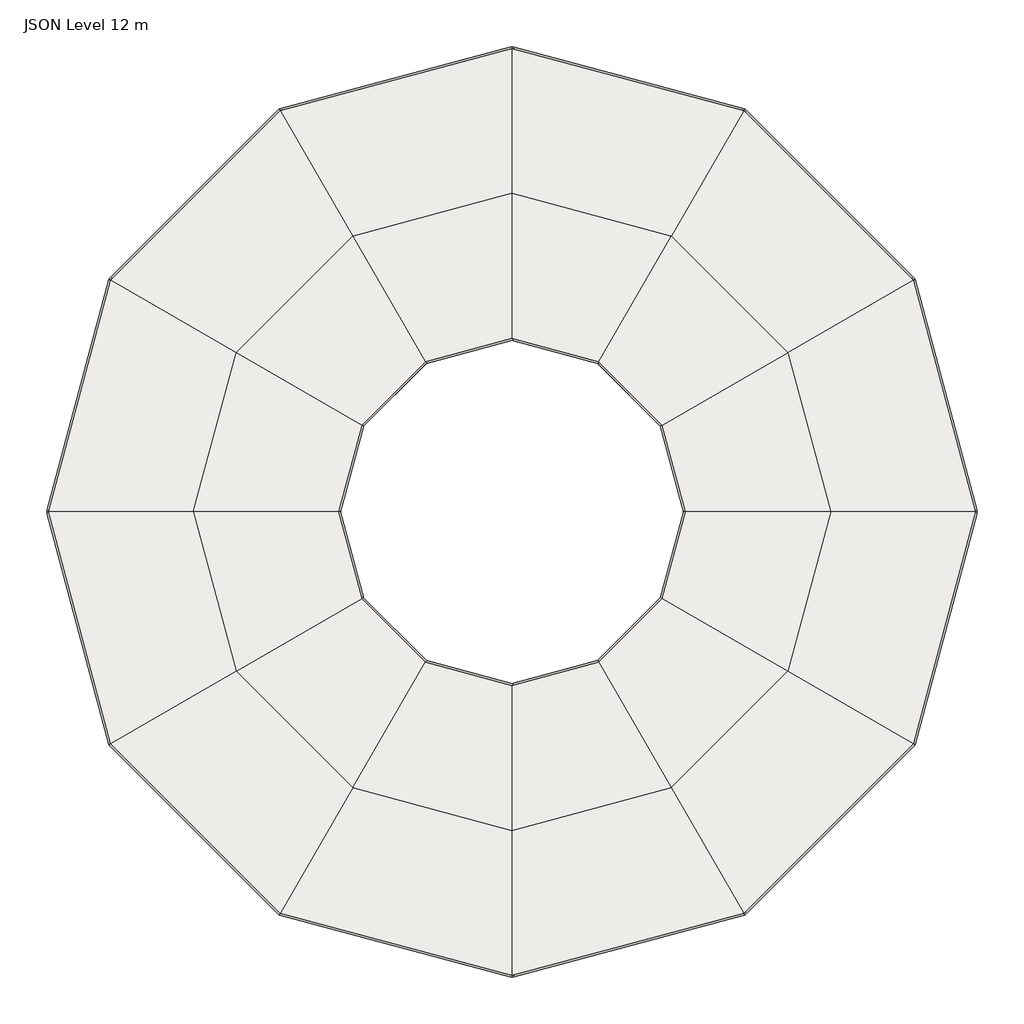
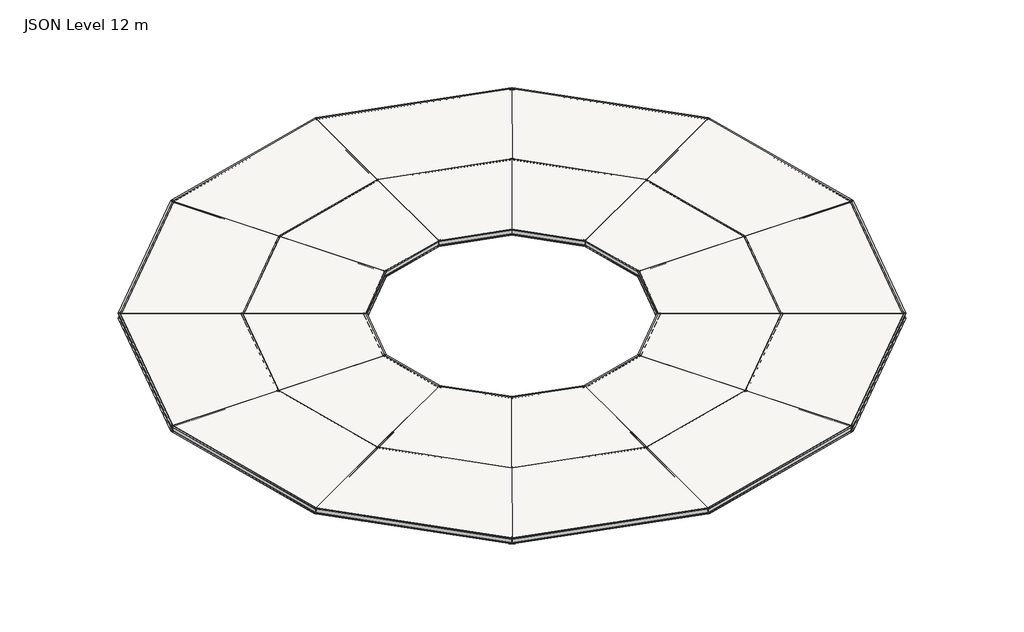
# One storey: 60 beams, 24 slabs.
"""IFC4 building model written with IfcOpenShell, lengths in millimetres."""

import ifcopenshell
import ifcopenshell.guid

model = None  # the IFC model being written
_history = None  # IfcOwnerHistory: only IFC2X3 demands one
_inside = {}  # id of a spatial element -> (the spatial element, [elements in it])
_under = {}  # id of a project, library or spatial element -> (it, [spatial elements below it])
_declared = {}  # id of a project -> (the project, [libraries it declares])
_typed = {}  # id of a type object -> (the type object, [elements of that type])
_made_of = {}  # id of a material, layer set ... -> (it, [elements and type objects made of it])


def new_model(schema):
    """Start an empty IFC model of exactly this schema.

    Asked for "IFC4X3", IfcOpenShell would pick the latest addendum, in which some entities
    have other attributes; the version numbers below select the first issue.
    IFC2X3 requires an IfcOwnerHistory on every rooted entity: one is made here for all.
    """
    global model, _history
    if schema == "IFC4X3":
        model = ifcopenshell.file(schema_version=(4, 3, 0, 0))
    else:
        model = ifcopenshell.file(schema=schema)
    _inside.clear()
    _under.clear()
    _declared.clear()
    _typed.clear()
    _made_of.clear()
    _history = None
    if model.schema == "IFC2X3":
        org = make("IfcOrganization", Name="unknown")
        user = make(
            "IfcPersonAndOrganization",
            ThePerson=make("IfcPerson", FamilyName="unknown"),
            TheOrganization=org,
        )
        app = make(
            "IfcApplication",
            ApplicationDeveloper=org,
            Version="unknown",
            ApplicationFullName="unknown",
            ApplicationIdentifier="unknown",
        )
        _history = make(
            "IfcOwnerHistory",
            OwningUser=user,
            OwningApplication=app,
            ChangeAction="ADDED",
            CreationDate=0,
        )
    return model


def make(cls, **values):
    """One entity of the class cls with the attributes given. An attribute that is None is left unset."""
    return model.create_entity(
        cls, **{name: value for name, value in values.items() if value is not None}
    )


def rooted(cls, **values):
    """An entity with a GlobalId (a new one), such as an element, a storey or a relation."""
    return make(cls, GlobalId=ifcopenshell.guid.new(), OwnerHistory=_history, **values)


def si_unit(unit_type, name, prefix=None):
    """IfcSIUnit, for example si_unit("LENGTHUNIT", "METRE", prefix="MILLI")."""
    return make("IfcSIUnit", UnitType=unit_type, Prefix=prefix, Name=name)


def assignment(units):
    """IfcUnitAssignment: the units of a project."""
    return None if units is None else make("IfcUnitAssignment", Units=units)


def point(xyz):
    """IfcCartesianPoint."""
    return None if xyz is None else make("IfcCartesianPoint", Coordinates=xyz)


def direction(xyz):
    """IfcDirection."""
    return None if xyz is None else make("IfcDirection", DirectionRatios=xyz)


def frame(location, z_axis=None, x_axis=None):
    """IfcAxis2Placement3D, a coordinate frame: its origin and axes. An axis left out is left unset."""
    return make(
        "IfcAxis2Placement3D",
        Location=point(location),
        Axis=direction(z_axis),
        RefDirection=direction(x_axis),
    )


def frame_2d(location, x_axis=None):
    """IfcAxis2Placement2D, a coordinate frame in the plane: its origin and x axis."""
    return make(
        "IfcAxis2Placement2D", Location=point(location), RefDirection=direction(x_axis)
    )


def origin():
    """The frame at (0, 0, 0) with its axes left unset."""
    return frame((0.0, 0.0, 0.0))


def place(relative_to, where):
    """IfcLocalPlacement: puts the frame where relative to a parent placement (None: the world)."""
    return make(
        "IfcLocalPlacement", PlacementRelTo=relative_to, RelativePlacement=where
    )


def context(
    kind, dimensions, precision=None, world=None, true_north=None, identifier=None
):
    """IfcGeometricRepresentationContext, for example the 3D "Model" context."""
    return make(
        "IfcGeometricRepresentationContext",
        ContextIdentifier=identifier,
        ContextType=kind,
        CoordinateSpaceDimension=dimensions,
        Precision=precision,
        WorldCoordinateSystem=world,
        TrueNorth=true_north,
    )


def project(units=None, contexts=None):
    """IfcProject with its units and contexts."""
    return rooted(
        "IfcProject",
        Name="project",
        RepresentationContexts=contexts,
        UnitsInContext=assignment(units),
    )


def spatial(cls, under=None, at=None, **own):
    """A site, building, storey or space (cls), placed at a placement, below another one or the project."""
    s = rooted(cls, ObjectPlacement=at, **own)
    if under is not None:
        _under.setdefault(under.id(), (under, []))[1].append(s)
    return s


def polyline(points):
    """IfcPolyline through the points."""
    return make("IfcPolyline", Points=[point(p) for p in points])


def circle_curve(where, radius):
    """IfcCircle in the frame where."""
    return make("IfcCircle", Position=where, Radius=radius)


def trimmed(basis, trim1, trim2, sense, master):
    """IfcTrimmedCurve: the piece of a basis curve between two trims."""
    return make(
        "IfcTrimmedCurve",
        BasisCurve=basis,
        Trim1=trim1,
        Trim2=trim2,
        SenseAgreement=sense,
        MasterRepresentation=master,
    )


def segment(curve, same_sense, transition):
    """IfcCompositeCurveSegment."""
    return make(
        "IfcCompositeCurveSegment",
        Transition=transition,
        SameSense=same_sense,
        ParentCurve=curve,
    )


def composite_curve(segments, self_intersect=None):
    """IfcCompositeCurve: segments joined end to end."""
    return make("IfcCompositeCurve", Segments=segments, SelfIntersect=self_intersect)


def outline(outer, holes=None, kind="AREA"):
    """IfcArbitraryClosedProfileDef: a profile drawn as a closed curve; with holes, ...WithVoids."""
    if holes is None:
        return make("IfcArbitraryClosedProfileDef", ProfileType=kind, OuterCurve=outer)
    return make(
        "IfcArbitraryProfileDefWithVoids",
        ProfileType=kind,
        OuterCurve=outer,
        InnerCurves=holes,
    )


def extrude(swept, where, along, depth):
    """IfcExtrudedAreaSolid: the profile swept, set in the frame where, extruded along a direction by depth."""
    return make(
        "IfcExtrudedAreaSolid",
        SweptArea=swept,
        Position=where,
        ExtrudedDirection=direction(along),
        Depth=depth,
    )


def shape(context_of_items, identifier, shape_type, items):
    """IfcShapeRepresentation: the items that make up one representation, for example the "Body"."""
    return make(
        "IfcShapeRepresentation",
        ContextOfItems=context_of_items,
        RepresentationIdentifier=identifier,
        RepresentationType=shape_type,
        Items=items,
    )


def source(mapping_origin, context_of_items, identifier, shape_type, items):
    """IfcRepresentationMap: a shape defined once, which mapped items show again and again."""
    return make(
        "IfcRepresentationMap",
        MappingOrigin=mapping_origin,
        MappedRepresentation=shape(context_of_items, identifier, shape_type, items),
    )


def transform(
    local_origin,
    x_axis=None,
    y_axis=None,
    z_axis=None,
    scale=None,
    scale2=None,
    scale3=None,
    uniform=True,
):
    """IfcCartesianTransformationOperator3D, or its non-uniform kind. x_axis, y_axis, z_axis: its Axis1, 2, 3."""
    if uniform:
        return make(
            "IfcCartesianTransformationOperator3D",
            Axis1=direction(x_axis),
            Axis2=direction(y_axis),
            LocalOrigin=point(local_origin),
            Scale=scale,
            Axis3=direction(z_axis),
        )
    return make(
        "IfcCartesianTransformationOperator3DnonUniform",
        Axis1=direction(x_axis),
        Axis2=direction(y_axis),
        LocalOrigin=point(local_origin),
        Scale=scale,
        Axis3=direction(z_axis),
        Scale2=scale2,
        Scale3=scale3,
    )


def mapped(mapping_source, mapping_target):
    """IfcMappedItem: shows the shape of a source again, moved by a transform."""
    return make(
        "IfcMappedItem", MappingSource=mapping_source, MappingTarget=mapping_target
    )


def made_of(thing, what):
    """Note that an element or type object is made of a material, layer set ...; save() writes the relation."""
    if what is not None:
        _made_of.setdefault(what.id(), (what, []))[1].append(thing)
    return thing


def element(
    cls,
    number,
    at=None,
    inside=None,
    cuts=None,
    type_object=None,
    material=None,
    context=None,
    identifier="Body",
    shape_type=None,
    held_by="IfcProductDefinitionShape",
    body=None,
    shapes=None,
    **own,
):
    """One element of the class cls, such as IfcWall. Its Tag is "e" and its number.

    at: its placement. inside: the storey or other place that contains it. cuts: it is an
    opening in that element (IfcRelVoidsElement). A single representation is given by context,
    identifier, shape_type and body (its items); several are given by shapes. held_by: the class
    of the entity that holds the representations. save() writes the other relations.
    """
    e = rooted(cls, Tag="e%d" % number, ObjectPlacement=at, **own)
    if body is not None:
        shapes = [shape(context, identifier, shape_type, body)]
    if shapes is not None:
        e.Representation = make(held_by, Representations=shapes)
    if inside is not None:
        _inside.setdefault(inside.id(), (inside, []))[1].append(e)
    if cuts is not None:
        rooted(
            "IfcRelVoidsElement", RelatingBuildingElement=cuts, RelatedOpeningElement=e
        )
    if type_object is not None:
        _typed.setdefault(type_object.id(), (type_object, []))[1].append(e)
    return made_of(e, material)


def aggregate(whole, parts):
    """IfcRelAggregates: a whole, such as a stair, and the parts it consists of."""
    return rooted("IfcRelAggregates", RelatingObject=whole, RelatedObjects=parts)


def save(model, path):
    """Write the relations noted so far, then the file.

    IfcRelAggregates (storeys below a building ...), IfcRelContainedInSpatialStructure (elements
    in a storey), IfcRelDefinesByType, IfcRelAssociatesMaterial and IfcRelDeclares: one each for
    every whole, place, type object, material and project.
    """
    for whole, parts in _under.values():
        aggregate(whole, parts)
    for where, things in _inside.values():
        rooted(
            "IfcRelContainedInSpatialStructure",
            RelatedElements=things,
            RelatingStructure=where,
        )
    for kind, things in _typed.values():
        rooted("IfcRelDefinesByType", RelatedObjects=things, RelatingType=kind)
    for what, things in _made_of.values():
        rooted("IfcRelAssociatesMaterial", RelatedObjects=things, RelatingMaterial=what)
    for by, libraries in _declared.values():
        rooted("IfcRelDeclares", RelatingContext=by, RelatedDefinitions=libraries)
    model.write(path)


def ub_universal_beams_ub254x146x31_beafa172(model_context):
    return source(origin(), model_context, "Body", "SweptSolid", [
        extrude(outline(composite_curve([segment(polyline([(73.05, -117.1), (73.05, -125.7), (-73.05, -125.7), (-73.05, -117.1), (-10.6, -117.1)]), True, "CONTINUOUS"), segment(trimmed(circle_curve(frame_2d((-10.6, -109.5)), 7.6), [point((-10.6, -117.1))], [point((-3.0, -109.5))], True, "CARTESIAN"), True, "CONTINUOUS"), segment(polyline([(-3.0, -109.5), (-3.0, 109.5)]), True, "CONTINUOUS"), segment(trimmed(circle_curve(frame_2d((-10.6, 109.5)), 7.6), [point((-3.0, 109.5))], [point((-10.6, 117.1))], True, "CARTESIAN"), True, "CONTINUOUS"), segment(polyline([(-10.6, 117.1), (-73.05, 117.1), (-73.05, 125.7), (73.05, 125.7), (73.05, 117.1), (10.6, 117.1)]), True, "CONTINUOUS"), segment(trimmed(circle_curve(frame_2d((10.6, 109.5)), 7.6), [point((10.6, 117.1))], [point((3.0, 109.5))], True, "CARTESIAN"), True, "CONTINUOUS"), segment(polyline([(3.0, 109.5), (3.0, -109.5)]), True, "CONTINUOUS"), segment(trimmed(circle_curve(frame_2d((10.6, -109.5)), 7.6), [point((3.0, -109.5))], [point((10.6, -117.1))], True, "CARTESIAN"), True, "CONTINUOUS"), segment(polyline([(10.6, -117.1), (73.05, -117.1)]), True, "CONTINUOUS")], self_intersect=False)), frame((-1552.9, 0.0, 0.0), z_axis=(1.0, 0.0, 0.0), x_axis=(0.0, 1.0, 0.0)), (0.0, 0.0, 1.0), 3105.8),
    ])


def ub_universal_beams_ub254x146x31_048477c2(model_context):
    return source(origin(), model_context, "Body", "SweptSolid", [
        extrude(outline(composite_curve([segment(polyline([(73.05, -117.1), (73.05, -125.7), (-73.05, -125.7), (-73.05, -117.1), (-10.6, -117.1)]), True, "CONTINUOUS"), segment(trimmed(circle_curve(frame_2d((-10.6, -109.5)), 7.6), [point((-10.6, -117.1))], [point((-3.0, -109.5))], True, "CARTESIAN"), True, "CONTINUOUS"), segment(polyline([(-3.0, -109.5), (-3.0, 109.5)]), True, "CONTINUOUS"), segment(trimmed(circle_curve(frame_2d((-10.6, 109.5)), 7.6), [point((-3.0, 109.5))], [point((-10.6, 117.1))], True, "CARTESIAN"), True, "CONTINUOUS"), segment(polyline([(-10.6, 117.1), (-73.05, 117.1), (-73.05, 125.7), (73.05, 125.7), (73.05, 117.1), (10.6, 117.1)]), True, "CONTINUOUS"), segment(trimmed(circle_curve(frame_2d((10.6, 109.5)), 7.6), [point((10.6, 117.1))], [point((3.0, 109.5))], True, "CARTESIAN"), True, "CONTINUOUS"), segment(polyline([(3.0, 109.5), (3.0, -109.5)]), True, "CONTINUOUS"), segment(trimmed(circle_curve(frame_2d((10.6, -109.5)), 7.6), [point((3.0, -109.5))], [point((10.6, -117.1))], True, "CARTESIAN"), True, "CONTINUOUS"), segment(polyline([(10.6, -117.1), (73.05, -117.1)]), True, "CONTINUOUS")], self_intersect=False)), frame((-2847.0, 0.0, 0.0), z_axis=(1.0, 0.0, 0.0), x_axis=(0.0, 1.0, 0.0)), (0.0, 0.0, 1.0), 5694.0),
    ])


def ub_universal_beams_ub254x146x31_9e4386c4(model_context):
    return source(origin(), model_context, "Body", "SweptSolid", [
        extrude(outline(composite_curve([segment(polyline([(73.05, -117.1), (73.05, -125.7), (-73.05, -125.7), (-73.05, -117.1), (-10.6, -117.1)]), True, "CONTINUOUS"), segment(trimmed(circle_curve(frame_2d((-10.6, -109.5)), 7.6), [point((-10.6, -117.1))], [point((-3.0, -109.5))], True, "CARTESIAN"), True, "CONTINUOUS"), segment(polyline([(-3.0, -109.5), (-3.0, 109.5)]), True, "CONTINUOUS"), segment(trimmed(circle_curve(frame_2d((-10.6, 109.5)), 7.6), [point((-3.0, 109.5))], [point((-10.6, 117.1))], True, "CARTESIAN"), True, "CONTINUOUS"), segment(polyline([(-10.6, 117.1), (-73.05, 117.1), (-73.05, 125.7), (73.05, 125.7), (73.05, 117.1), (10.6, 117.1)]), True, "CONTINUOUS"), segment(trimmed(circle_curve(frame_2d((10.6, 109.5)), 7.6), [point((10.6, 117.1))], [point((3.0, 109.5))], True, "CARTESIAN"), True, "CONTINUOUS"), segment(polyline([(3.0, 109.5), (3.0, -109.5)]), True, "CONTINUOUS"), segment(trimmed(circle_curve(frame_2d((10.6, -109.5)), 7.6), [point((3.0, -109.5))], [point((10.6, -117.1))], True, "CARTESIAN"), True, "CONTINUOUS"), segment(polyline([(10.6, -117.1), (73.05, -117.1)]), True, "CONTINUOUS")], self_intersect=False)), frame((-4141.1, 0.0, 0.0), z_axis=(1.0, 0.0, 0.0), x_axis=(0.0, 1.0, 0.0)), (0.0, 0.0, 1.0), 8282.2),
    ])


def ub_universal_beams_ub254x146x31_ce116be2(model_context):
    return source(origin(), model_context, "Body", "SweptSolid", [
        extrude(outline(composite_curve([segment(polyline([(73.05, -117.1), (73.05, -125.7), (-73.05, -125.7), (-73.05, -117.1), (-10.6, -117.1)]), True, "CONTINUOUS"), segment(trimmed(circle_curve(frame_2d((-10.6, -109.5)), 7.6), [point((-10.6, -117.1))], [point((-3.0, -109.5))], True, "CARTESIAN"), True, "CONTINUOUS"), segment(polyline([(-3.0, -109.5), (-3.0, 109.5)]), True, "CONTINUOUS"), segment(trimmed(circle_curve(frame_2d((-10.6, 109.5)), 7.6), [point((-3.0, 109.5))], [point((-10.6, 117.1))], True, "CARTESIAN"), True, "CONTINUOUS"), segment(polyline([(-10.6, 117.1), (-73.05, 117.1), (-73.05, 125.7), (73.05, 125.7), (73.05, 117.1), (10.6, 117.1)]), True, "CONTINUOUS"), segment(trimmed(circle_curve(frame_2d((10.6, 109.5)), 7.6), [point((10.6, 117.1))], [point((3.0, 109.5))], True, "CARTESIAN"), True, "CONTINUOUS"), segment(polyline([(3.0, 109.5), (3.0, -109.5)]), True, "CONTINUOUS"), segment(trimmed(circle_curve(frame_2d((10.6, -109.5)), 7.6), [point((3.0, -109.5))], [point((10.6, -117.1))], True, "CARTESIAN"), True, "CONTINUOUS"), segment(polyline([(10.6, -117.1), (73.05, -117.1)]), True, "CONTINUOUS")], self_intersect=False)), frame((-2500.0, 0.0, 0.0), z_axis=(1.0, 0.0, 0.0), x_axis=(0.0, 1.0, 0.0)), (0.0, 0.0, 1.0), 5000.0),
    ])


model = new_model("IFC4")

# Units and contexts
model_context = context("Model", 3, world=origin())
ifc_project = project(units=[si_unit("LENGTHUNIT", "METRE", prefix="MILLI")], contexts=[model_context])

# Site, building, storey
site = spatial("IfcSite", under=ifc_project)
building = spatial("IfcBuilding", under=site)
storey = spatial("IfcBuildingStorey", under=building, Name="JSON Level 12 m", Elevation=12000.0)

# Beams
placement = place(None, origin())
ub_universal_beams_ub254x146x31_shape = ub_universal_beams_ub254x146x31_beafa172(model_context)
element("IfcBeam", 1, ObjectType="UB-Universal Beams : UB254x146x31", at=placement, inside=storey, context=model_context, shape_type="MappedRepresentation", body=[
    mapped(ub_universal_beams_ub254x146x31_shape, transform((5598.0762114, 1500.0, 11874.3), x_axis=(-0.2588190451025206, 0.9659258262890683, 0.0), y_axis=(-0.9659258262890683, -0.2588190451025206, 0.0), z_axis=(0.0, 0.0, 1.0))),
])
element("IfcBeam", 2, ObjectType="UB-Universal Beams : UB254x146x31", at=placement, inside=storey, context=model_context, shape_type="MappedRepresentation", body=[
    mapped(ub_universal_beams_ub254x146x31_shape, transform((4098.0762114, 4098.0762114, 11874.3), x_axis=(-0.7071067811865472, 0.7071067811865477, 0.0), y_axis=(-0.7071067811865477, -0.7071067811865472, 0.0), z_axis=(0.0, 0.0, 1.0))),
])
element("IfcBeam", 3, ObjectType="UB-Universal Beams : UB254x146x31", at=placement, inside=storey, context=model_context, shape_type="MappedRepresentation", body=[
    mapped(ub_universal_beams_ub254x146x31_shape, transform((1500.0, 5598.0762114, 11874.3), x_axis=(-0.9659258262890683, 0.2588190451025205, 0.0), y_axis=(-0.2588190451025205, -0.9659258262890683, 0.0), z_axis=(0.0, 0.0, 1.0))),
])
element("IfcBeam", 4, ObjectType="UB-Universal Beams : UB254x146x31", at=placement, inside=storey, context=model_context, shape_type="MappedRepresentation", body=[
    mapped(ub_universal_beams_ub254x146x31_shape, transform((-1500.0, 5598.0762114, 11874.3), x_axis=(-0.9659258262890683, -0.2588190451025206, 0.0), y_axis=(0.2588190451025206, -0.9659258262890683, 0.0), z_axis=(0.0, 0.0, 1.0))),
])
element("IfcBeam", 5, ObjectType="UB-Universal Beams : UB254x146x31", at=placement, inside=storey, context=model_context, shape_type="MappedRepresentation", body=[
    mapped(ub_universal_beams_ub254x146x31_shape, transform((-4098.0762114, 4098.0762114, 11874.3), x_axis=(-0.7071067811865477, -0.7071067811865475, 0.0), y_axis=(0.7071067811865475, -0.7071067811865477, 0.0), z_axis=(0.0, 0.0, 1.0))),
])
element("IfcBeam", 6, ObjectType="UB-Universal Beams : UB254x146x31", at=placement, inside=storey, context=model_context, shape_type="MappedRepresentation", body=[
    mapped(ub_universal_beams_ub254x146x31_shape, transform((-5598.0762114, 1500.0, 11874.3), x_axis=(-0.25881904510252063, -0.9659258262890683, 0.0), y_axis=(0.9659258262890683, -0.25881904510252063, 0.0), z_axis=(0.0, 0.0, 1.0))),
])
element("IfcBeam", 7, ObjectType="UB-Universal Beams : UB254x146x31", at=placement, inside=storey, context=model_context, shape_type="MappedRepresentation", body=[
    mapped(ub_universal_beams_ub254x146x31_shape, transform((-5598.0762114, -1500.0, 11874.3), x_axis=(0.25881904510252035, -0.9659258262890685, 0.0), y_axis=(0.9659258262890685, 0.25881904510252035, 0.0), z_axis=(0.0, 0.0, 1.0))),
])
element("IfcBeam", 8, ObjectType="UB-Universal Beams : UB254x146x31", at=placement, inside=storey, context=model_context, shape_type="MappedRepresentation", body=[
    mapped(ub_universal_beams_ub254x146x31_shape, transform((-4098.0762114, -4098.0762114, 11874.3), x_axis=(0.7071067811865471, -0.7071067811865478, 0.0), y_axis=(0.7071067811865478, 0.7071067811865471, 0.0), z_axis=(0.0, 0.0, 1.0))),
])
element("IfcBeam", 9, ObjectType="UB-Universal Beams : UB254x146x31", at=placement, inside=storey, context=model_context, shape_type="MappedRepresentation", body=[
    mapped(ub_universal_beams_ub254x146x31_shape, transform((-1500.0, -5598.0762114, 11874.3), x_axis=(0.9659258262890682, -0.25881904510252074, 0.0), y_axis=(0.25881904510252074, 0.9659258262890682, 0.0), z_axis=(0.0, 0.0, 1.0))),
])
element("IfcBeam", 10, ObjectType="UB-Universal Beams : UB254x146x31", at=placement, inside=storey, context=model_context, shape_type="MappedRepresentation", body=[
    mapped(ub_universal_beams_ub254x146x31_shape, transform((1500.0, -5598.0762114, 11874.3), x_axis=(0.9659258262890684, 0.25881904510252035, 0.0), y_axis=(-0.25881904510252035, 0.9659258262890684, 0.0), z_axis=(0.0, 0.0, 1.0))),
])
element("IfcBeam", 11, ObjectType="UB-Universal Beams : UB254x146x31", at=placement, inside=storey, context=model_context, shape_type="MappedRepresentation", body=[
    mapped(ub_universal_beams_ub254x146x31_shape, transform((4098.0762114, -4098.0762114, 11874.3), x_axis=(0.7071067811865474, 0.7071067811865476, 0.0), y_axis=(-0.7071067811865476, 0.7071067811865474, 0.0), z_axis=(0.0, 0.0, 1.0))),
])
element("IfcBeam", 12, ObjectType="UB-Universal Beams : UB254x146x31", at=placement, inside=storey, context=model_context, shape_type="MappedRepresentation", body=[
    mapped(ub_universal_beams_ub254x146x31_shape, transform((5598.0762114, -1500.0, 11874.3), x_axis=(0.25881904510252096, 0.9659258262890682, 0.0), y_axis=(-0.9659258262890682, 0.25881904510252096, 0.0), z_axis=(0.0, 0.0, 1.0))),
])
ub_universal_beams_ub254x146x31_2_shape = ub_universal_beams_ub254x146x31_048477c2(model_context)
element("IfcBeam", 13, ObjectType="UB-Universal Beams : UB254x146x31", at=placement, inside=storey, context=model_context, shape_type="MappedRepresentation", body=[
    mapped(ub_universal_beams_ub254x146x31_2_shape, transform((10263.1397208, 2750.0, 11874.3), x_axis=(-0.2588190451025204, 0.9659258262890684, 0.0), y_axis=(-0.9659258262890684, -0.2588190451025204, 0.0), z_axis=(0.0, 0.0, 1.0))),
])
element("IfcBeam", 14, ObjectType="UB-Universal Beams : UB254x146x31", at=placement, inside=storey, context=model_context, shape_type="MappedRepresentation", body=[
    mapped(ub_universal_beams_ub254x146x31_2_shape, transform((7513.1397208, 7513.1397208, 11874.3), x_axis=(-0.7071067811865476, 0.7071067811865476, 0.0), y_axis=(-0.7071067811865476, -0.7071067811865476, 0.0), z_axis=(0.0, 0.0, 1.0))),
])
element("IfcBeam", 15, ObjectType="UB-Universal Beams : UB254x146x31", at=placement, inside=storey, context=model_context, shape_type="MappedRepresentation", body=[
    mapped(ub_universal_beams_ub254x146x31_2_shape, transform((2750.0, 10263.1397208, 11874.3), x_axis=(-0.9659258262890682, 0.2588190451025207, 0.0), y_axis=(-0.2588190451025207, -0.9659258262890682, 0.0), z_axis=(0.0, 0.0, 1.0))),
])
element("IfcBeam", 16, ObjectType="UB-Universal Beams : UB254x146x31", at=placement, inside=storey, context=model_context, shape_type="MappedRepresentation", body=[
    mapped(ub_universal_beams_ub254x146x31_2_shape, transform((-2750.0, 10263.1397208, 11874.3), x_axis=(-0.9659258262890684, -0.2588190451025204, 0.0), y_axis=(0.2588190451025204, -0.9659258262890684, 0.0), z_axis=(0.0, 0.0, 1.0))),
])
element("IfcBeam", 17, ObjectType="UB-Universal Beams : UB254x146x31", at=placement, inside=storey, context=model_context, shape_type="MappedRepresentation", body=[
    mapped(ub_universal_beams_ub254x146x31_2_shape, transform((-7513.1397208, 7513.1397208, 11874.3), x_axis=(-0.7071067811865476, -0.7071067811865475, 0.0), y_axis=(0.7071067811865475, -0.7071067811865476, 0.0), z_axis=(0.0, 0.0, 1.0))),
])
element("IfcBeam", 18, ObjectType="UB-Universal Beams : UB254x146x31", at=placement, inside=storey, context=model_context, shape_type="MappedRepresentation", body=[
    mapped(ub_universal_beams_ub254x146x31_2_shape, transform((-10263.1397208, 2750.0, 11874.3), x_axis=(-0.25881904510252046, -0.9659258262890684, 0.0), y_axis=(0.9659258262890684, -0.25881904510252046, 0.0), z_axis=(0.0, 0.0, 1.0))),
])
element("IfcBeam", 19, ObjectType="UB-Universal Beams : UB254x146x31", at=placement, inside=storey, context=model_context, shape_type="MappedRepresentation", body=[
    mapped(ub_universal_beams_ub254x146x31_2_shape, transform((-10263.1397208, -2750.0, 11874.3), x_axis=(0.2588190451025204, -0.9659258262890684, 0.0), y_axis=(0.9659258262890684, 0.2588190451025204, 0.0), z_axis=(0.0, 0.0, 1.0))),
])
element("IfcBeam", 20, ObjectType="UB-Universal Beams : UB254x146x31", at=placement, inside=storey, context=model_context, shape_type="MappedRepresentation", body=[
    mapped(ub_universal_beams_ub254x146x31_2_shape, transform((-7513.1397208, -7513.1397208, 11874.3), x_axis=(0.7071067811865472, -0.7071067811865478, 0.0), y_axis=(0.7071067811865478, 0.7071067811865472, 0.0), z_axis=(0.0, 0.0, 1.0))),
])
element("IfcBeam", 21, ObjectType="UB-Universal Beams : UB254x146x31", at=placement, inside=storey, context=model_context, shape_type="MappedRepresentation", body=[
    mapped(ub_universal_beams_ub254x146x31_2_shape, transform((-2750.0, -10263.1397208, 11874.3), x_axis=(0.9659258262890682, -0.2588190451025209, 0.0), y_axis=(0.2588190451025209, 0.9659258262890682, 0.0), z_axis=(0.0, 0.0, 1.0))),
])
element("IfcBeam", 22, ObjectType="UB-Universal Beams : UB254x146x31", at=placement, inside=storey, context=model_context, shape_type="MappedRepresentation", body=[
    mapped(ub_universal_beams_ub254x146x31_2_shape, transform((2750.0, -10263.1397208, 11874.3), x_axis=(0.9659258262890682, 0.2588190451025205, 0.0), y_axis=(-0.2588190451025205, 0.9659258262890682, 0.0), z_axis=(0.0, 0.0, 1.0))),
])
element("IfcBeam", 23, ObjectType="UB-Universal Beams : UB254x146x31", at=placement, inside=storey, context=model_context, shape_type="MappedRepresentation", body=[
    mapped(ub_universal_beams_ub254x146x31_2_shape, transform((7513.1397208, -7513.1397208, 11874.3), x_axis=(0.7071067811865478, 0.7071067811865474, 0.0), y_axis=(-0.7071067811865474, 0.7071067811865478, 0.0), z_axis=(0.0, 0.0, 1.0))),
])
element("IfcBeam", 24, ObjectType="UB-Universal Beams : UB254x146x31", at=placement, inside=storey, context=model_context, shape_type="MappedRepresentation", body=[
    mapped(ub_universal_beams_ub254x146x31_2_shape, transform((10263.1397208, -2750.0, 11874.3), x_axis=(0.2588190451025208, 0.9659258262890682, 0.0), y_axis=(-0.9659258262890682, 0.2588190451025208, 0.0), z_axis=(0.0, 0.0, 1.0))),
])
ub_universal_beams_ub254x146x31_3_shape = ub_universal_beams_ub254x146x31_9e4386c4(model_context)
element("IfcBeam", 25, ObjectType="UB-Universal Beams : UB254x146x31", at=placement, inside=storey, context=model_context, shape_type="MappedRepresentation", body=[
    mapped(ub_universal_beams_ub254x146x31_3_shape, transform((14928.2032303, 4000.0, 11874.3), x_axis=(-0.2588190451025207, 0.9659258262890683, 0.0), y_axis=(-0.9659258262890683, -0.2588190451025207, 0.0), z_axis=(0.0, 0.0, 1.0))),
])
element("IfcBeam", 26, ObjectType="UB-Universal Beams : UB254x146x31", at=placement, inside=storey, context=model_context, shape_type="MappedRepresentation", body=[
    mapped(ub_universal_beams_ub254x146x31_3_shape, transform((10928.2032303, 10928.2032303, 11874.3), x_axis=(-0.7071067811865475, 0.7071067811865476, 0.0), y_axis=(-0.7071067811865476, -0.7071067811865475, 0.0), z_axis=(0.0, 0.0, 1.0))),
])
element("IfcBeam", 27, ObjectType="UB-Universal Beams : UB254x146x31", at=placement, inside=storey, context=model_context, shape_type="MappedRepresentation", body=[
    mapped(ub_universal_beams_ub254x146x31_3_shape, transform((4000.0, 14928.2032303, 11874.3), x_axis=(-0.9659258262890682, 0.25881904510252085, 0.0), y_axis=(-0.25881904510252085, -0.9659258262890682, 0.0), z_axis=(0.0, 0.0, 1.0))),
])
element("IfcBeam", 28, ObjectType="UB-Universal Beams : UB254x146x31", at=placement, inside=storey, context=model_context, shape_type="MappedRepresentation", body=[
    mapped(ub_universal_beams_ub254x146x31_3_shape, transform((-4000.0, 14928.2032303, 11874.3), x_axis=(-0.9659258262890683, -0.2588190451025207, 0.0), y_axis=(0.2588190451025207, -0.9659258262890683, 0.0), z_axis=(0.0, 0.0, 1.0))),
])
element("IfcBeam", 29, ObjectType="UB-Universal Beams : UB254x146x31", at=placement, inside=storey, context=model_context, shape_type="MappedRepresentation", body=[
    mapped(ub_universal_beams_ub254x146x31_3_shape, transform((-10928.2032303, 10928.2032303, 11874.3), x_axis=(-0.7071067811865477, -0.7071067811865474, 0.0), y_axis=(0.7071067811865474, -0.7071067811865477, 0.0), z_axis=(0.0, 0.0, 1.0))),
])
element("IfcBeam", 30, ObjectType="UB-Universal Beams : UB254x146x31", at=placement, inside=storey, context=model_context, shape_type="MappedRepresentation", body=[
    mapped(ub_universal_beams_ub254x146x31_3_shape, transform((-14928.2032303, 4000.0, 11874.3), x_axis=(-0.25881904510252074, -0.9659258262890683, 0.0), y_axis=(0.9659258262890683, -0.25881904510252074, 0.0), z_axis=(0.0, 0.0, 1.0))),
])
element("IfcBeam", 31, ObjectType="UB-Universal Beams : UB254x146x31", at=placement, inside=storey, context=model_context, shape_type="MappedRepresentation", body=[
    mapped(ub_universal_beams_ub254x146x31_3_shape, transform((-14928.2032303, -4000.0, 11874.3), x_axis=(0.25881904510252046, -0.9659258262890683, 0.0), y_axis=(0.9659258262890683, 0.25881904510252046, 0.0), z_axis=(0.0, 0.0, 1.0))),
])
element("IfcBeam", 32, ObjectType="UB-Universal Beams : UB254x146x31", at=placement, inside=storey, context=model_context, shape_type="MappedRepresentation", body=[
    mapped(ub_universal_beams_ub254x146x31_3_shape, transform((-10928.2032303, -10928.2032303, 11874.3), x_axis=(0.7071067811865472, -0.7071067811865479, 0.0), y_axis=(0.7071067811865479, 0.7071067811865472, 0.0), z_axis=(0.0, 0.0, 1.0))),
])
element("IfcBeam", 33, ObjectType="UB-Universal Beams : UB254x146x31", at=placement, inside=storey, context=model_context, shape_type="MappedRepresentation", body=[
    mapped(ub_universal_beams_ub254x146x31_3_shape, transform((-4000.0, -14928.2032303, 11874.3), x_axis=(0.9659258262890682, -0.25881904510252096, 0.0), y_axis=(0.25881904510252096, 0.9659258262890682, 0.0), z_axis=(0.0, 0.0, 1.0))),
])
element("IfcBeam", 34, ObjectType="UB-Universal Beams : UB254x146x31", at=placement, inside=storey, context=model_context, shape_type="MappedRepresentation", body=[
    mapped(ub_universal_beams_ub254x146x31_3_shape, transform((4000.0, -14928.2032303, 11874.3), x_axis=(0.9659258262890684, 0.25881904510252074, 0.0), y_axis=(-0.25881904510252074, 0.9659258262890684, 0.0), z_axis=(0.0, 0.0, 1.0))),
])
element("IfcBeam", 35, ObjectType="UB-Universal Beams : UB254x146x31", at=placement, inside=storey, context=model_context, shape_type="MappedRepresentation", body=[
    mapped(ub_universal_beams_ub254x146x31_3_shape, transform((10928.2032303, -10928.2032303, 11874.3), x_axis=(0.7071067811865476, 0.7071067811865475, 0.0), y_axis=(-0.7071067811865475, 0.7071067811865476, 0.0), z_axis=(0.0, 0.0, 1.0))),
])
element("IfcBeam", 36, ObjectType="UB-Universal Beams : UB254x146x31", at=placement, inside=storey, context=model_context, shape_type="MappedRepresentation", body=[
    mapped(ub_universal_beams_ub254x146x31_3_shape, transform((14928.2032303, -4000.0, 11874.3), x_axis=(0.25881904510252113, 0.9659258262890682, 0.0), y_axis=(-0.9659258262890682, 0.25881904510252113, 0.0), z_axis=(0.0, 0.0, 1.0))),
])
ub_universal_beams_ub254x146x31_4_shape = ub_universal_beams_ub254x146x31_ce116be2(model_context)
element("IfcBeam", 37, ObjectType="UB-Universal Beams : UB254x146x31", at=placement, inside=storey, context=model_context, shape_type="MappedRepresentation", body=[
    mapped(ub_universal_beams_ub254x146x31_4_shape, transform((8500.0, 0.0, 11874.3), x_axis=(1.0, 0.0, 0.0), y_axis=(0.0, 1.0, 0.0), z_axis=(0.0, 0.0, 1.0))),
])
element("IfcBeam", 38, ObjectType="UB-Universal Beams : UB254x146x31", at=placement, inside=storey, context=model_context, shape_type="MappedRepresentation", body=[
    mapped(ub_universal_beams_ub254x146x31_4_shape, transform((13500.0, 0.0, 11874.3), x_axis=(1.0, 0.0, 0.0), y_axis=(0.0, 1.0, 0.0), z_axis=(0.0, 0.0, 1.0))),
])
element("IfcBeam", 39, ObjectType="UB-Universal Beams : UB254x146x31", at=placement, inside=storey, context=model_context, shape_type="MappedRepresentation", body=[
    mapped(ub_universal_beams_ub254x146x31_4_shape, transform((7361.2159322, 4250.0, 11874.3), x_axis=(0.8660254037844388, 0.4999999999999998, 0.0), y_axis=(-0.4999999999999998, 0.8660254037844388, 0.0), z_axis=(0.0, 0.0, 1.0))),
])
element("IfcBeam", 40, ObjectType="UB-Universal Beams : UB254x146x31", at=placement, inside=storey, context=model_context, shape_type="MappedRepresentation", body=[
    mapped(ub_universal_beams_ub254x146x31_4_shape, transform((11691.3429511, 6750.0, 11874.3), x_axis=(0.8660254037844386, 0.5000000000000001, 0.0), y_axis=(-0.5000000000000001, 0.8660254037844386, 0.0), z_axis=(0.0, 0.0, 1.0))),
])
element("IfcBeam", 41, ObjectType="UB-Universal Beams : UB254x146x31", at=placement, inside=storey, context=model_context, shape_type="MappedRepresentation", body=[
    mapped(ub_universal_beams_ub254x146x31_4_shape, transform((4250.0, 7361.2159322, 11874.3), x_axis=(0.5, 0.8660254037844386, 0.0), y_axis=(-0.8660254037844386, 0.5, 0.0), z_axis=(0.0, 0.0, 1.0))),
])
element("IfcBeam", 42, ObjectType="UB-Universal Beams : UB254x146x31", at=placement, inside=storey, context=model_context, shape_type="MappedRepresentation", body=[
    mapped(ub_universal_beams_ub254x146x31_4_shape, transform((6750.0, 11691.3429511, 11874.3), x_axis=(0.5000000000000002, 0.8660254037844384, 0.0), y_axis=(-0.8660254037844384, 0.5000000000000002, 0.0), z_axis=(0.0, 0.0, 1.0))),
])
element("IfcBeam", 43, ObjectType="UB-Universal Beams : UB254x146x31", at=placement, inside=storey, context=model_context, shape_type="MappedRepresentation", body=[
    mapped(ub_universal_beams_ub254x146x31_4_shape, transform((0.0, 8500.0, 11874.3), x_axis=(0.0, 1.0, 0.0), y_axis=(-1.0, 0.0, 0.0), z_axis=(0.0, 0.0, 1.0))),
])
element("IfcBeam", 44, ObjectType="UB-Universal Beams : UB254x146x31", at=placement, inside=storey, context=model_context, shape_type="MappedRepresentation", body=[
    mapped(ub_universal_beams_ub254x146x31_4_shape, transform((0.0, 13500.0, 11874.3), x_axis=(0.0, 1.0, 0.0), y_axis=(-1.0, 0.0, 0.0), z_axis=(0.0, 0.0, 1.0))),
])
element("IfcBeam", 45, ObjectType="UB-Universal Beams : UB254x146x31", at=placement, inside=storey, context=model_context, shape_type="MappedRepresentation", body=[
    mapped(ub_universal_beams_ub254x146x31_4_shape, transform((-4250.0, 7361.2159322, 11874.3), x_axis=(-0.49999999999999967, 0.8660254037844388, 0.0), y_axis=(-0.8660254037844388, -0.49999999999999967, 0.0), z_axis=(0.0, 0.0, 1.0))),
])
element("IfcBeam", 46, ObjectType="UB-Universal Beams : UB254x146x31", at=placement, inside=storey, context=model_context, shape_type="MappedRepresentation", body=[
    mapped(ub_universal_beams_ub254x146x31_4_shape, transform((-6750.0, 11691.3429511, 11874.3), x_axis=(-0.4999999999999999, 0.8660254037844386, 0.0), y_axis=(-0.8660254037844386, -0.4999999999999999, 0.0), z_axis=(0.0, 0.0, 1.0))),
])
element("IfcBeam", 47, ObjectType="UB-Universal Beams : UB254x146x31", at=placement, inside=storey, context=model_context, shape_type="MappedRepresentation", body=[
    mapped(ub_universal_beams_ub254x146x31_4_shape, transform((-7361.2159322, 4250.0, 11874.3), x_axis=(-0.8660254037844388, 0.4999999999999998, 0.0), y_axis=(-0.4999999999999998, -0.8660254037844388, 0.0), z_axis=(0.0, 0.0, 1.0))),
])
element("IfcBeam", 48, ObjectType="UB-Universal Beams : UB254x146x31", at=placement, inside=storey, context=model_context, shape_type="MappedRepresentation", body=[
    mapped(ub_universal_beams_ub254x146x31_4_shape, transform((-11691.3429511, 6750.0, 11874.3), x_axis=(-0.8660254037844386, 0.5000000000000001, 0.0), y_axis=(-0.5000000000000001, -0.8660254037844386, 0.0), z_axis=(0.0, 0.0, 1.0))),
])
element("IfcBeam", 49, ObjectType="UB-Universal Beams : UB254x146x31", at=placement, inside=storey, context=model_context, shape_type="MappedRepresentation", body=[
    mapped(ub_universal_beams_ub254x146x31_4_shape, transform((-8500.0, 0.0, 11874.3), x_axis=(-1.0, 0.0, 0.0), y_axis=(0.0, -1.0, 0.0), z_axis=(0.0, 0.0, 1.0))),
])
element("IfcBeam", 50, ObjectType="UB-Universal Beams : UB254x146x31", at=placement, inside=storey, context=model_context, shape_type="MappedRepresentation", body=[
    mapped(ub_universal_beams_ub254x146x31_4_shape, transform((-13500.0, 0.0, 11874.3), x_axis=(-1.0, 0.0, 0.0), y_axis=(0.0, -1.0, 0.0), z_axis=(0.0, 0.0, 1.0))),
])
element("IfcBeam", 51, ObjectType="UB-Universal Beams : UB254x146x31", at=placement, inside=storey, context=model_context, shape_type="MappedRepresentation", body=[
    mapped(ub_universal_beams_ub254x146x31_4_shape, transform((-7361.2159322, -4250.0, 11874.3), x_axis=(-0.8660254037844388, -0.4999999999999999, 0.0), y_axis=(0.4999999999999999, -0.8660254037844388, 0.0), z_axis=(0.0, 0.0, 1.0))),
])
element("IfcBeam", 52, ObjectType="UB-Universal Beams : UB254x146x31", at=placement, inside=storey, context=model_context, shape_type="MappedRepresentation", body=[
    mapped(ub_universal_beams_ub254x146x31_4_shape, transform((-11691.3429511, -6750.0, 11874.3), x_axis=(-0.8660254037844388, -0.49999999999999956, 0.0), y_axis=(0.49999999999999956, -0.8660254037844388, 0.0), z_axis=(0.0, 0.0, 1.0))),
])
element("IfcBeam", 53, ObjectType="UB-Universal Beams : UB254x146x31", at=placement, inside=storey, context=model_context, shape_type="MappedRepresentation", body=[
    mapped(ub_universal_beams_ub254x146x31_4_shape, transform((-4250.0, -7361.2159322, 11874.3), x_axis=(-0.5000000000000006, -0.8660254037844384, 0.0), y_axis=(0.8660254037844384, -0.5000000000000006, 0.0), z_axis=(0.0, 0.0, 1.0))),
])
element("IfcBeam", 54, ObjectType="UB-Universal Beams : UB254x146x31", at=placement, inside=storey, context=model_context, shape_type="MappedRepresentation", body=[
    mapped(ub_universal_beams_ub254x146x31_4_shape, transform((-6750.0, -11691.3429511, 11874.3), x_axis=(-0.5000000000000004, -0.8660254037844384, 0.0), y_axis=(0.8660254037844384, -0.5000000000000004, 0.0), z_axis=(0.0, 0.0, 1.0))),
])
element("IfcBeam", 55, ObjectType="UB-Universal Beams : UB254x146x31", at=placement, inside=storey, context=model_context, shape_type="MappedRepresentation", body=[
    mapped(ub_universal_beams_ub254x146x31_4_shape, transform((0.0, -8500.0, 11874.3), x_axis=(0.0, -1.0, 0.0), y_axis=(1.0, 0.0, 0.0), z_axis=(0.0, 0.0, 1.0))),
])
element("IfcBeam", 56, ObjectType="UB-Universal Beams : UB254x146x31", at=placement, inside=storey, context=model_context, shape_type="MappedRepresentation", body=[
    mapped(ub_universal_beams_ub254x146x31_4_shape, transform((0.0, -13500.0, 11874.3), x_axis=(0.0, -1.0, 0.0), y_axis=(1.0, 0.0, 0.0), z_axis=(0.0, 0.0, 1.0))),
])
element("IfcBeam", 57, ObjectType="UB-Universal Beams : UB254x146x31", at=placement, inside=storey, context=model_context, shape_type="MappedRepresentation", body=[
    mapped(ub_universal_beams_ub254x146x31_4_shape, transform((4250.0, -7361.2159322, 11874.3), x_axis=(0.5, -0.8660254037844386, 0.0), y_axis=(0.8660254037844386, 0.5, 0.0), z_axis=(0.0, 0.0, 1.0))),
])
element("IfcBeam", 58, ObjectType="UB-Universal Beams : UB254x146x31", at=placement, inside=storey, context=model_context, shape_type="MappedRepresentation", body=[
    mapped(ub_universal_beams_ub254x146x31_4_shape, transform((6750.0, -11691.3429511, 11874.3), x_axis=(0.5000000000000002, -0.8660254037844384, 0.0), y_axis=(0.8660254037844384, 0.5000000000000002, 0.0), z_axis=(0.0, 0.0, 1.0))),
])
element("IfcBeam", 59, ObjectType="UB-Universal Beams : UB254x146x31", at=placement, inside=storey, context=model_context, shape_type="MappedRepresentation", body=[
    mapped(ub_universal_beams_ub254x146x31_4_shape, transform((7361.2159322, -4250.0, 11874.3), x_axis=(0.8660254037844384, -0.5000000000000004, 0.0), y_axis=(0.5000000000000004, 0.8660254037844384, 0.0), z_axis=(0.0, 0.0, 1.0))),
])
element("IfcBeam", 60, ObjectType="UB-Universal Beams : UB254x146x31", at=placement, inside=storey, context=model_context, shape_type="MappedRepresentation", body=[
    mapped(ub_universal_beams_ub254x146x31_4_shape, transform((11691.3429511, -6750.0, 11874.3), x_axis=(0.8660254037844384, -0.5000000000000007, 0.0), y_axis=(0.5000000000000007, 0.8660254037844384, 0.0), z_axis=(0.0, 0.0, 1.0))),
])

# Slabs
element("IfcSlab", 61, ObjectType="Concrete 150mm", at=placement, inside=storey, context=model_context, shape_type="SweptSolid", body=[
    extrude(outline(polyline([(11000.0, 0.0), (6000.0, 0.0), (5196.1524227, 3000.0), (9526.2794416, 5500.0), (11000.0, 0.0)])), frame((0.0, 0.0, 11850.0), z_axis=(0.0, 0.0, 1.0), x_axis=(1.0, 0.0, 0.0)), (0.0, 0.0, 1.0), 150.0),
])
element("IfcSlab", 62, ObjectType="Concrete 150mm", at=placement, inside=storey, context=model_context, shape_type="SweptSolid", body=[
    extrude(outline(polyline([(9526.2794416, 5500.0), (5196.1524227, 3000.0), (3000.0, 5196.1524227), (5500.0, 9526.2794416), (9526.2794416, 5500.0)])), frame((0.0, 0.0, 11850.0), z_axis=(0.0, 0.0, 1.0), x_axis=(1.0, 0.0, 0.0)), (0.0, 0.0, 1.0), 150.0),
])
element("IfcSlab", 63, ObjectType="Concrete 150mm", at=placement, inside=storey, context=model_context, shape_type="SweptSolid", body=[
    extrude(outline(polyline([(5500.0, 9526.2794416), (3000.0, 5196.1524227), (0.0, 6000.0), (0.0, 11000.0), (5500.0, 9526.2794416)])), frame((0.0, 0.0, 11850.0), z_axis=(0.0, 0.0, 1.0), x_axis=(1.0, 0.0, 0.0)), (0.0, 0.0, 1.0), 150.0),
])
element("IfcSlab", 64, ObjectType="Concrete 150mm", at=placement, inside=storey, context=model_context, shape_type="SweptSolid", body=[
    extrude(outline(polyline([(0.0, 11000.0), (0.0, 6000.0), (-3000.0, 5196.1524227), (-5500.0, 9526.2794416), (0.0, 11000.0)])), frame((0.0, 0.0, 11850.0), z_axis=(0.0, 0.0, 1.0), x_axis=(1.0, 0.0, 0.0)), (0.0, 0.0, 1.0), 150.0),
])
element("IfcSlab", 65, ObjectType="Concrete 150mm", at=placement, inside=storey, context=model_context, shape_type="SweptSolid", body=[
    extrude(outline(polyline([(-5500.0, 9526.2794416), (-3000.0, 5196.1524227), (-5196.1524227, 3000.0), (-9526.2794416, 5500.0), (-5500.0, 9526.2794416)])), frame((0.0, 0.0, 11850.0), z_axis=(0.0, 0.0, 1.0), x_axis=(1.0, 0.0, 0.0)), (0.0, 0.0, 1.0), 150.0),
])
element("IfcSlab", 66, ObjectType="Concrete 150mm", at=placement, inside=storey, context=model_context, shape_type="SweptSolid", body=[
    extrude(outline(polyline([(-9526.2794416, 5500.0), (-5196.1524227, 3000.0), (-6000.0, 0.0), (-11000.0, 0.0), (-9526.2794416, 5500.0)])), frame((0.0, 0.0, 11850.0), z_axis=(0.0, 0.0, 1.0), x_axis=(1.0, 0.0, 0.0)), (0.0, 0.0, 1.0), 150.0),
])
element("IfcSlab", 67, ObjectType="Concrete 150mm", at=placement, inside=storey, context=model_context, shape_type="SweptSolid", body=[
    extrude(outline(polyline([(-11000.0, 0.0), (-6000.0, 0.0), (-5196.1524227, -3000.0), (-9526.2794416, -5500.0), (-11000.0, 0.0)])), frame((0.0, 0.0, 11850.0), z_axis=(0.0, 0.0, 1.0), x_axis=(1.0, 0.0, 0.0)), (0.0, 0.0, 1.0), 150.0),
])
element("IfcSlab", 68, ObjectType="Concrete 150mm", at=placement, inside=storey, context=model_context, shape_type="SweptSolid", body=[
    extrude(outline(polyline([(-9526.2794416, -5500.0), (-5196.1524227, -3000.0), (-3000.0, -5196.1524227), (-5500.0, -9526.2794416), (-9526.2794416, -5500.0)])), frame((0.0, 0.0, 11850.0), z_axis=(0.0, 0.0, 1.0), x_axis=(1.0, 0.0, 0.0)), (0.0, 0.0, 1.0), 150.0),
])
element("IfcSlab", 69, ObjectType="Concrete 150mm", at=placement, inside=storey, context=model_context, shape_type="SweptSolid", body=[
    extrude(outline(polyline([(-5500.0, -9526.2794416), (-3000.0, -5196.1524227), (0.0, -6000.0), (0.0, -11000.0), (-5500.0, -9526.2794416)])), frame((0.0, 0.0, 11850.0), z_axis=(0.0, 0.0, 1.0), x_axis=(1.0, 0.0, 0.0)), (0.0, 0.0, 1.0), 150.0),
])
element("IfcSlab", 70, ObjectType="Concrete 150mm", at=placement, inside=storey, context=model_context, shape_type="SweptSolid", body=[
    extrude(outline(polyline([(0.0, -11000.0), (0.0, -6000.0), (3000.0, -5196.1524227), (5500.0, -9526.2794416), (0.0, -11000.0)])), frame((0.0, 0.0, 11850.0), z_axis=(0.0, 0.0, 1.0), x_axis=(1.0, 0.0, 0.0)), (0.0, 0.0, 1.0), 150.0),
])
element("IfcSlab", 71, ObjectType="Concrete 150mm", at=placement, inside=storey, context=model_context, shape_type="SweptSolid", body=[
    extrude(outline(polyline([(5500.0, -9526.2794416), (3000.0, -5196.1524227), (5196.1524227, -3000.0), (9526.2794416, -5500.0), (5500.0, -9526.2794416)])), frame((0.0, 0.0, 11850.0), z_axis=(0.0, 0.0, 1.0), x_axis=(1.0, 0.0, 0.0)), (0.0, 0.0, 1.0), 150.0),
])
element("IfcSlab", 72, ObjectType="Concrete 150mm", at=placement, inside=storey, context=model_context, shape_type="SweptSolid", body=[
    extrude(outline(polyline([(9526.2794416, -5500.0), (5196.1524227, -3000.0), (6000.0, 0.0), (11000.0, 0.0), (9526.2794416, -5500.0)])), frame((0.0, 0.0, 11850.0), z_axis=(0.0, 0.0, 1.0), x_axis=(1.0, 0.0, 0.0)), (0.0, 0.0, 1.0), 150.0),
])
element("IfcSlab", 73, ObjectType="Concrete 150mm", at=placement, inside=storey, context=model_context, shape_type="SweptSolid", body=[
    extrude(outline(polyline([(16000.0, 0.0), (11000.0, 0.0), (9526.2794416, 5500.0), (13856.4064606, 8000.0), (16000.0, 0.0)])), frame((0.0, 0.0, 11850.0), z_axis=(0.0, 0.0, 1.0), x_axis=(1.0, 0.0, 0.0)), (0.0, 0.0, 1.0), 150.0),
])
element("IfcSlab", 74, ObjectType="Concrete 150mm", at=placement, inside=storey, context=model_context, shape_type="SweptSolid", body=[
    extrude(outline(polyline([(13856.4064606, 8000.0), (9526.2794416, 5500.0), (5500.0, 9526.2794416), (8000.0, 13856.4064606), (13856.4064606, 8000.0)])), frame((0.0, 0.0, 11850.0), z_axis=(0.0, 0.0, 1.0), x_axis=(1.0, 0.0, 0.0)), (0.0, 0.0, 1.0), 150.0),
])
element("IfcSlab", 75, ObjectType="Concrete 150mm", at=placement, inside=storey, context=model_context, shape_type="SweptSolid", body=[
    extrude(outline(polyline([(8000.0, 13856.4064606), (5500.0, 9526.2794416), (0.0, 11000.0), (0.0, 16000.0), (8000.0, 13856.4064606)])), frame((0.0, 0.0, 11850.0), z_axis=(0.0, 0.0, 1.0), x_axis=(1.0, 0.0, 0.0)), (0.0, 0.0, 1.0), 150.0),
])
element("IfcSlab", 76, ObjectType="Concrete 150mm", at=placement, inside=storey, context=model_context, shape_type="SweptSolid", body=[
    extrude(outline(polyline([(0.0, 16000.0), (0.0, 11000.0), (-5500.0, 9526.2794416), (-8000.0, 13856.4064606), (0.0, 16000.0)])), frame((0.0, 0.0, 11850.0), z_axis=(0.0, 0.0, 1.0), x_axis=(1.0, 0.0, 0.0)), (0.0, 0.0, 1.0), 150.0),
])
element("IfcSlab", 77, ObjectType="Concrete 150mm", at=placement, inside=storey, context=model_context, shape_type="SweptSolid", body=[
    extrude(outline(polyline([(-8000.0, 13856.4064606), (-5500.0, 9526.2794416), (-9526.2794416, 5500.0), (-13856.4064606, 8000.0), (-8000.0, 13856.4064606)])), frame((0.0, 0.0, 11850.0), z_axis=(0.0, 0.0, 1.0), x_axis=(1.0, 0.0, 0.0)), (0.0, 0.0, 1.0), 150.0),
])
element("IfcSlab", 78, ObjectType="Concrete 150mm", at=placement, inside=storey, context=model_context, shape_type="SweptSolid", body=[
    extrude(outline(polyline([(-13856.4064606, 8000.0), (-9526.2794416, 5500.0), (-11000.0, 0.0), (-16000.0, 0.0), (-13856.4064606, 8000.0)])), frame((0.0, 0.0, 11850.0), z_axis=(0.0, 0.0, 1.0), x_axis=(1.0, 0.0, 0.0)), (0.0, 0.0, 1.0), 150.0),
])
element("IfcSlab", 79, ObjectType="Concrete 150mm", at=placement, inside=storey, context=model_context, shape_type="SweptSolid", body=[
    extrude(outline(polyline([(-16000.0, 0.0), (-11000.0, 0.0), (-9526.2794416, -5500.0), (-13856.4064606, -8000.0), (-16000.0, 0.0)])), frame((0.0, 0.0, 11850.0), z_axis=(0.0, 0.0, 1.0), x_axis=(1.0, 0.0, 0.0)), (0.0, 0.0, 1.0), 150.0),
])
element("IfcSlab", 80, ObjectType="Concrete 150mm", at=placement, inside=storey, context=model_context, shape_type="SweptSolid", body=[
    extrude(outline(polyline([(-13856.4064606, -8000.0), (-9526.2794416, -5500.0), (-5500.0, -9526.2794416), (-8000.0, -13856.4064606), (-13856.4064606, -8000.0)])), frame((0.0, 0.0, 11850.0), z_axis=(0.0, 0.0, 1.0), x_axis=(1.0, 0.0, 0.0)), (0.0, 0.0, 1.0), 150.0),
])
element("IfcSlab", 81, ObjectType="Concrete 150mm", at=placement, inside=storey, context=model_context, shape_type="SweptSolid", body=[
    extrude(outline(polyline([(-8000.0, -13856.4064606), (-5500.0, -9526.2794416), (0.0, -11000.0), (0.0, -16000.0), (-8000.0, -13856.4064606)])), frame((0.0, 0.0, 11850.0), z_axis=(0.0, 0.0, 1.0), x_axis=(1.0, 0.0, 0.0)), (0.0, 0.0, 1.0), 150.0),
])
element("IfcSlab", 82, ObjectType="Concrete 150mm", at=placement, inside=storey, context=model_context, shape_type="SweptSolid", body=[
    extrude(outline(polyline([(0.0, -16000.0), (0.0, -11000.0), (5500.0, -9526.2794416), (8000.0, -13856.4064606), (0.0, -16000.0)])), frame((0.0, 0.0, 11850.0), z_axis=(0.0, 0.0, 1.0), x_axis=(1.0, 0.0, 0.0)), (0.0, 0.0, 1.0), 150.0),
])
element("IfcSlab", 83, ObjectType="Concrete 150mm", at=placement, inside=storey, context=model_context, shape_type="SweptSolid", body=[
    extrude(outline(polyline([(8000.0, -13856.4064606), (5500.0, -9526.2794416), (9526.2794416, -5500.0), (13856.4064606, -8000.0), (8000.0, -13856.4064606)])), frame((0.0, 0.0, 11850.0), z_axis=(0.0, 0.0, 1.0), x_axis=(1.0, 0.0, 0.0)), (0.0, 0.0, 1.0), 150.0),
])
element("IfcSlab", 84, ObjectType="Concrete 150mm", at=placement, inside=storey, context=model_context, shape_type="SweptSolid", body=[
    extrude(outline(polyline([(13856.4064606, -8000.0), (9526.2794416, -5500.0), (11000.0, 0.0), (16000.0, 0.0), (13856.4064606, -8000.0)])), frame((0.0, 0.0, 11850.0), z_axis=(0.0, 0.0, 1.0), x_axis=(1.0, 0.0, 0.0)), (0.0, 0.0, 1.0), 150.0),
])

save(model, "model.ifc")

# Revit data of these elements
# Type "UB-Universal Beams : UB254x146x31"
#   Section Name Key = "UB254X146X31"
#   Width = 14.61 cm
#   Web Thickness = 0.6 cm
#   Web Fillet = 0.76 cm
#   Warping Constant = 66000.0 cm⁶
#   Torsional Moment of Inertia = 8.55 cm⁴
#   Section Area = 39.7 cm²
#   Plastic Modulus weak axis = 94.1 cm³
#   Plastic Modulus strong axis = 393.0 cm³
#   Nominal Weight = 31.10 kgf/m
#   Moment of Inertia weak axis = 448.00 cm⁴
#   Moment of Inertia strong axis = 4413.00 cm⁴
#   Height = 25.14 cm
#   Flange Thickness = 0.86 cm
#   Elastic Modulus weak axis = 61.3 cm³
#   Elastic Modulus strong axis = 351.0 cm³
#   Centroid Vertical = 12.57 cm
#   Centroid Horizontal = 7.305 cm
#   Bolt Spacing = 7.0 cm
#   Length [instance default] = 1500 mm
#   Structural Material [instance default] = Metal - Steel 43-275
#   Type Comments = ""
#   Assembly Code = ""
# Type "Concrete 150mm"
#   Description = "Concrete Floor, 100mm thick, Interior Function"
#   Assembly Code = "B1010"
#   Type Mark = "SF01"
#   Function = 0
#   Layers, outside or top first: 150 mm "Concrete, Cast-in-Place gray" (function 1)
# Elements 1, 2, 3, 4, 5, 6, 7, 8, 9, 10, 11, 12, 13, 14, 15, 16, 17, 18, 19, 20, 21, 22, 23, 24, 25, 26, 27, 28, 29, 30, 31, 32, 33, 34, 35, 36, 37, 38, 39, 40, 41, 42, 43, 44, 45, 46, 47, 48, 49, 50, 51, 52, 53, 54, 55, 56, 57, 58, 59, 60 (IfcBeam, "UB-Universal Beams : UB254x146x31")
#   Structural Material = Metal - Steel 43-275
#   Phase Created = New Construction
#   Materials on its faces: "Metal - Steel 43-275"
# Elements 61, 62, 63, 64, 65, 66, 67, 68, 69, 70, 71, 72, 73, 74, 75, 76, 77, 78, 79, 80, 81, 82, 83, 84 (IfcSlab, "Concrete 150mm")
#   Height Offset From Level = 0 mm
#   built-in parameter 1001954 = 1
#   Phase Created = New Construction
#   Materials on its faces: "Concrete, Cast-in-Place gray"
# Materials
#   "Metal - Steel 43-275": class "Metal", colour RGB 247 247 247, transparency 0, Cost = 0
#   "Concrete, Cast-in-Place gray": class "Concrete", colour RGB 192 192 192, transparency 0, Description = "Cast-in-place concrete", Cost = 0
